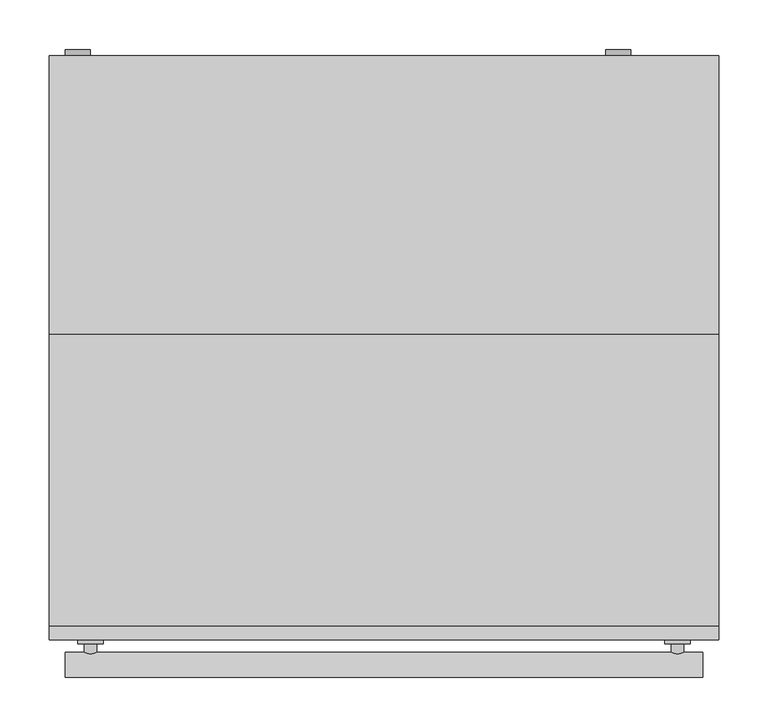
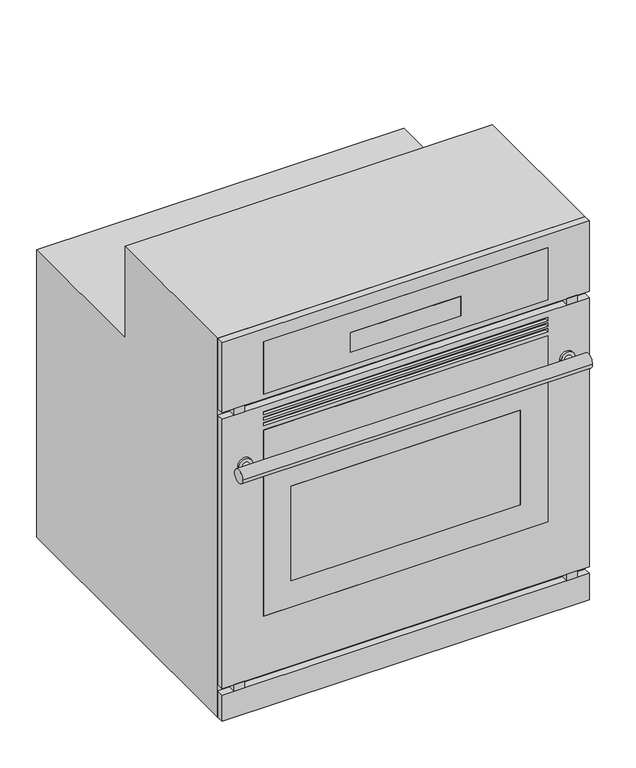
"""IFC4 building model written with IfcOpenShell, lengths in millimetres: proxy geometry, Ovens_Built-In-Wall-Single_GE-Monogram_ZEK938SMSS : Ovens_Built-In-Wall-Single_GE-Monogram_ZEK938SMSS."""

from ifc_helpers import new_model, si_unit, point, frame, frame_2d, origin, place, context, project, spatial, polyline, circle_curve, trimmed, segment, composite_curve, outline, extrude, faceted_brep, source, transform, mapped, element, save
from ifc_brep_helpers import plane_surface, cylinder_surface, advanced_brep


def specialty_equipment_95a57712(model_context):
    return source(origin(), model_context, "Body", "SolidModel", [
        advanced_brep(
        [(-309.3357143, -313.0409311, 485.7987745), (-283.9357143, -313.0409311, 485.7987745), (-290.2857143, -313.0409311, 485.7987745), (-302.9857143, -313.0409311, 485.7987745), (-309.3357143, -308.7303349, 485.7987745), (-283.9357143, -308.7303349, 485.7987745), (-302.9857143, -334.1303349, 485.7987745), (-290.2857143, -334.1303349, 485.7987745)],
        [
            (0, 1, circle_curve(frame((-296.6357143, -313.0409311, 485.7987745), z_axis=(0.0, -1.0, 0.0), x_axis=(1.0, 0.0, 0.0)), 12.7)),
            (1, 0, circle_curve(frame((-296.6357143, -313.0409311, 485.7987745), z_axis=(0.0, -1.0, 0.0), x_axis=(1.0, 0.0, 0.0)), 12.7)),
            (2, 3, circle_curve(frame((-296.6357143, -313.0409311, 485.7987745), z_axis=(0.0, 1.0, 0.0), x_axis=(1.0, 0.0, 0.0)), 6.35)),
            (3, 2, circle_curve(frame((-296.6357143, -313.0409311, 485.7987745), z_axis=(0.0, 1.0, 0.0), x_axis=(1.0, 0.0, 0.0)), 6.35)),
            (4, 5, circle_curve(frame((-296.6357143, -308.7303349, 485.7987745), z_axis=(0.0, 1.0, 0.0), x_axis=(1.0, 0.0, 0.0)), 12.7)),
            (5, 4, circle_curve(frame((-296.6357143, -308.7303349, 485.7987745), z_axis=(0.0, 1.0, 0.0), x_axis=(1.0, 0.0, 0.0)), 12.7)),
            (0, 4),
            (5, 1),
            (6, 7, circle_curve(frame((-296.6357143, -334.1303349, 485.7987745), z_axis=(0.0, -1.0, 0.0), x_axis=(1.0, 0.0, 0.0)), 6.35)),
            (7, 6, circle_curve(frame((-296.6357143, -334.1303349, 485.7987745), z_axis=(0.0, -1.0, 0.0), x_axis=(1.0, 0.0, 0.0)), 6.35)),
            (6, 3),
            (2, 7),
        ],
        [
            plane_surface(frame((-283.9357143, -313.0409311, 485.7987745), z_axis=(0.0, -1.0, 0.0), x_axis=(0.0, 0.0, 1.0))),
            plane_surface(frame((-283.9357143, -308.7303349, 485.7987745), z_axis=(0.0, 1.0, 0.0), x_axis=(0.0, 0.0, -1.0))),
            cylinder_surface(frame((-296.6357143, -308.7303349, 485.7987745), z_axis=(0.0, -1.0, 0.0), x_axis=(1.0, 0.0, 0.0)), 12.7),
            plane_surface(frame((-290.2857143, -334.1303349, 485.7987745), z_axis=(0.0, -1.0, 0.0), x_axis=(0.0, 0.0, 1.0))),
            cylinder_surface(frame((-296.6357143, -308.7303349, 485.7987745), z_axis=(0.0, -1.0, 0.0), x_axis=(1.0, 0.0, 0.0)), 6.35),
        ],
        [
            (0, [[1, 2], [3, 4]]),
            (1, [[5, 6]]),
            (2, [[-1, 7, -6, 8]]),
            (2, [[-2, -8, -5, -7]]),
            (3, [[9, 10]]),
            (4, [[-9, 11, -3, 12]]),
            (4, [[-10, -12, -4, -11]]),
        ],
    ),
        advanced_brep(
        [(283.9357143, -313.0409311, 485.7987745), (309.3357143, -313.0409311, 485.7987745), (302.9857143, -313.0409311, 485.7987745), (290.2857143, -313.0409311, 485.7987745), (283.9357143, -308.7303349, 485.7987745), (309.3357143, -308.7303349, 485.7987745), (290.2857143, -334.1303349, 485.7987745), (302.9857143, -334.1303349, 485.7987745)],
        [
            (0, 1, circle_curve(frame((296.6357143, -313.0409311, 485.7987745), z_axis=(0.0, -1.0, 0.0), x_axis=(1.0, 0.0, 0.0)), 12.7)),
            (1, 0, circle_curve(frame((296.6357143, -313.0409311, 485.7987745), z_axis=(0.0, -1.0, 0.0), x_axis=(1.0, 0.0, 0.0)), 12.7)),
            (2, 3, circle_curve(frame((296.6357143, -313.0409311, 485.7987745), z_axis=(0.0, 1.0, 0.0), x_axis=(1.0, 0.0, 0.0)), 6.35)),
            (3, 2, circle_curve(frame((296.6357143, -313.0409311, 485.7987745), z_axis=(0.0, 1.0, 0.0), x_axis=(1.0, 0.0, 0.0)), 6.35)),
            (4, 5, circle_curve(frame((296.6357143, -308.7303349, 485.7987745), z_axis=(0.0, 1.0, 0.0), x_axis=(1.0, 0.0, 0.0)), 12.7)),
            (5, 4, circle_curve(frame((296.6357143, -308.7303349, 485.7987745), z_axis=(0.0, 1.0, 0.0), x_axis=(1.0, 0.0, 0.0)), 12.7)),
            (0, 4),
            (5, 1),
            (6, 7, circle_curve(frame((296.6357143, -334.1303349, 485.7987745), z_axis=(0.0, -1.0, 0.0), x_axis=(1.0, 0.0, 0.0)), 6.35)),
            (7, 6, circle_curve(frame((296.6357143, -334.1303349, 485.7987745), z_axis=(0.0, -1.0, 0.0), x_axis=(1.0, 0.0, 0.0)), 6.35)),
            (6, 3),
            (2, 7),
        ],
        [
            plane_surface(frame((-283.9357143, -313.0409311, 485.7987745), z_axis=(0.0, -1.0, 0.0), x_axis=(0.0, 0.0, 1.0))),
            plane_surface(frame((-283.9357143, -308.7303349, 485.7987745), z_axis=(0.0, 1.0, 0.0), x_axis=(0.0, 0.0, -1.0))),
            cylinder_surface(frame((296.6357143, -308.7303349, 485.7987745), z_axis=(0.0, -1.0, 0.0), x_axis=(1.0, 0.0, 0.0)), 12.7),
            plane_surface(frame((-290.2857143, -334.1303349, 485.7987745), z_axis=(0.0, -1.0, 0.0), x_axis=(0.0, 0.0, 1.0))),
            cylinder_surface(frame((296.6357143, -308.7303349, 485.7987745), z_axis=(0.0, -1.0, 0.0), x_axis=(1.0, 0.0, 0.0)), 6.35),
        ],
        [
            (0, [[1, 2], [3, 4]]),
            (1, [[5, 6]]),
            (2, [[-1, 7, -6, 8]]),
            (2, [[-2, -8, -5, -7]]),
            (3, [[9, 10]]),
            (4, [[-9, 11, -3, 12]]),
            (4, [[-10, -12, -4, -11]]),
        ],
    ),
        extrude(outline(composite_curve([segment(trimmed(circle_curve(frame_2d((-334.1303349, 486.3026594)), 12.7), [point((-346.8303349, 486.3026594))], [point((-321.4303349, 486.3026594))], False, "CARTESIAN"), True, "CONTINUOUS"), segment(trimmed(circle_curve(frame_2d((-334.1303349, 486.3026594)), 12.7), [point((-321.4303349, 486.3026594))], [point((-346.8303349, 486.3026594))], False, "CARTESIAN"), True, "CONTINUOUS")], self_intersect=False)), frame((-322.0357143, 0.0, 0.0), z_axis=(1.0, 0.0, 0.0), x_axis=(0.0, 1.0, 0.0)), (0.0, 0.0, 1.0), 644.0714286),
        extrude(outline(polyline([(101.6, -308.7303349), (-101.6, -308.7303349), (-101.6, -295.275), (101.6, -295.275), (101.6, -308.7303349)])), frame((0.0, 0.0, 635.0), z_axis=(0.0, 0.0, 1.0), x_axis=(1.0, 0.0, 0.0)), (0.0, 0.0, 1.0), 38.1),
        extrude(outline(polyline([(211.1375, -308.7303349), (-211.1375, -308.7303349), (-211.1375, -295.275), (211.1375, -295.275), (211.1375, -308.7303349)])), frame((0.0, 0.0, 228.6), z_axis=(0.0, 0.0, 1.0), x_axis=(1.0, 0.0, 0.0)), (0.0, 0.0, 1.0), 184.15),
        extrude(outline(polyline([(711.2, 261.9375), (711.2, -261.9375), (609.6, -261.9375), (609.6, 261.9375), (711.2, 261.9375)]), holes=[polyline([(673.1, 101.6), (635.0, 101.6), (635.0, -101.6), (673.1, -101.6), (673.1, 101.6)])]), frame((0.0, -308.7303349, 0.0), z_axis=(0.0, 1.0, 0.0), x_axis=(0.0, 0.0, 1.0)), (0.0, 0.0, 1.0), 13.4553349),
        extrude(outline(polyline([(539.75, -261.9375), (177.8, -261.9375), (177.8, 261.9375), (539.75, 261.9375), (539.75, -261.9375)]), holes=[polyline([(228.6, 211.1375), (228.6, -211.1375), (412.75, -211.1375), (412.75, 211.1375), (228.6, 211.1375)])]), frame((0.0, -308.7303349, 0.0), z_axis=(0.0, 1.0, 0.0), x_axis=(0.0, 0.0, 1.0)), (0.0, 0.0, 1.0), 13.4553349),
        extrude(outline(polyline([(-296.970361, -308.7303349), (-316.020361, -308.7303349), (-316.020361, -295.275), (-296.970361, -295.275), (-296.970361, -308.7303349)])), frame((0.0, 0.0, 50.8), z_axis=(0.0, 0.0, 1.0), x_axis=(1.0, 0.0, 0.0)), (0.0, 0.0, 1.0), 12.7),
        extrude(outline(polyline([(316.020361, -308.7303349), (296.970361, -308.7303349), (296.970361, -295.275), (316.020361, -295.275), (316.020361, -308.7303349)])), frame((0.0, 0.0, 50.8), z_axis=(0.0, 0.0, 1.0), x_axis=(1.0, 0.0, 0.0)), (0.0, 0.0, 1.0), 12.7),
        extrude(outline(polyline([(-296.970361, -308.7303349), (-316.020361, -308.7303349), (-316.020361, -295.275), (-296.970361, -295.275), (-296.970361, -308.7303349)])), frame((0.0, 0.0, 587.3987745), z_axis=(0.0, 0.0, 1.0), x_axis=(1.0, 0.0, 0.0)), (0.0, 0.0, 1.0), 12.7),
        extrude(outline(polyline([(316.020361, -308.7303349), (296.970361, -308.7303349), (296.970361, -295.275), (316.020361, -295.275), (316.020361, -308.7303349)])), frame((0.0, 0.0, 587.3987745), z_axis=(0.0, 0.0, 1.0), x_axis=(1.0, 0.0, 0.0)), (0.0, 0.0, 1.0), 12.7),
        faceted_brep([(-338.1375, -308.7303349, 736.6), (-338.1375, -308.7303349, 600.0987745), (338.1375, -308.7303349, 600.0987745), (338.1375, -308.7303349, 736.6), (-261.9375, -308.7303349, 711.2), (261.9375, -308.7303349, 711.2), (261.9375, -308.7303349, 609.6), (-261.9375, -308.7303349, 609.6), (-338.1375, -295.275, 736.6), (338.1375, -295.275, 736.6), (338.1375, -295.275, 600.0987745), (-338.1375, -295.275, 600.0987745), (-261.9375, -295.275, 711.2), (-261.9375, -295.275, 609.6), (261.9375, -295.275, 609.6), (261.9375, -295.275, 711.2)], [[[0, 1, 2, 3], [4, 5, 6, 7]], [[8, 9, 10, 11], [12, 13, 14, 15]], [[1, 0, 8, 11]], [[2, 1, 11, 10]], [[3, 2, 10, 9]], [[0, 3, 9, 8]], [[5, 4, 12, 15]], [[6, 5, 15, 14]], [[7, 6, 14, 13]], [[4, 7, 13, 12]]]),
        faceted_brep([(338.1375, -308.7303349, 0.0), (338.1375, -308.7303349, 50.8), (-338.1375, -308.7303349, 50.8), (-338.1375, -308.7303349, 0.0), (338.1375, -295.275, 0.0), (-338.1375, -295.275, 0.0), (-338.1375, -295.275, 50.8), (338.1375, -295.275, 50.8)], [[[0, 1, 2, 3]], [[4, 5, 6, 7]], [[1, 0, 4, 7]], [[2, 1, 7, 6]], [[3, 2, 6, 5]], [[0, 3, 5, 4]]]),
        faceted_brep([(-338.1375, -308.7303349, 63.5), (338.1375, -308.7303349, 63.5), (338.1375, -308.7303349, 587.3987745), (-338.1375, -308.7303349, 587.3987745), (-261.9375, -308.7303349, 558.6731386), (-261.9375, -308.7303349, 565.0231386), (261.9375, -308.7303349, 565.0231386), (261.9375, -308.7303349, 558.6731386), (-261.9375, -308.7303349, 177.8), (-261.9375, -308.7303349, 539.75), (261.9375, -308.7303349, 539.75), (261.9375, -308.7303349, 177.8), (-261.9375, -308.7303349, 548.0044527), (-261.9375, -308.7303349, 554.3544527), (261.9375, -308.7303349, 554.3544527), (261.9375, -308.7303349, 548.0044527), (-261.9375, -308.7303349, 569.3418245), (-261.9375, -308.7303349, 575.6918245), (261.9375, -308.7303349, 575.6918245), (261.9375, -308.7303349, 569.3418245), (-338.1375, -295.275, 63.5), (-338.1375, -295.275, 587.3987745), (338.1375, -295.275, 587.3987745), (338.1375, -295.275, 63.5), (261.9375, -295.275, 177.8), (261.9375, -295.275, 539.75), (-261.9375, -295.275, 539.75), (-261.9375, -295.275, 177.8), (261.9375, -302.3803349, 565.0231386), (261.9375, -302.3803349, 558.6731386), (261.9375, -302.3803349, 554.3544527), (261.9375, -302.3803349, 548.0044527), (261.9375, -302.3803349, 575.6918245), (261.9375, -302.3803349, 569.3418245), (-261.9375, -302.3803349, 558.6731386), (-261.9375, -302.3803349, 565.0231386), (-261.9375, -302.3803349, 548.0044527), (-261.9375, -302.3803349, 554.3544527), (-261.9375, -302.3803349, 569.3418245), (-261.9375, -302.3803349, 575.6918245)], [[[0, 1, 2, 3], [4, 5, 6, 7], [8, 9, 10, 11], [12, 13, 14, 15], [16, 17, 18, 19]], [[20, 21, 22, 23], [24, 25, 26, 27]], [[1, 0, 20, 23]], [[2, 1, 23, 22]], [[3, 2, 22, 21]], [[7, 6, 28, 29]], [[15, 14, 30, 31]], [[19, 18, 32, 33]], [[24, 11, 10, 25]], [[8, 11, 24, 27]], [[5, 4, 34, 35]], [[13, 12, 36, 37]], [[17, 16, 38, 39]], [[8, 27, 26, 9]], [[0, 3, 21, 20]], [[18, 17, 39, 32]], [[32, 39, 38, 33]], [[33, 38, 16, 19]], [[6, 5, 35, 28]], [[28, 35, 34, 29]], [[29, 34, 4, 7]], [[14, 13, 37, 30]], [[30, 37, 36, 31]], [[31, 36, 12, 15]], [[26, 25, 10, 9]]]),
        extrude(outline(polyline([(-295.275, 0.0), (-295.275, 736.6), (0.0, 736.6), (0.0, 558.8), (281.8196651, 558.8), (281.8196651, 0.0), (-295.275, 0.0)])), frame((-338.1375, 0.0, 0.0), z_axis=(1.0, 0.0, 0.0), x_axis=(0.0, 1.0, 0.0)), (0.0, 0.0, 1.0), 676.275),
        extrude(outline(composite_curve([segment(trimmed(circle_curve(frame_2d((314.6288473, -309.3887314)), 12.7), [point((314.6288473, -296.6887314))], [point((314.6288473, -322.0887314))], False, "CARTESIAN"), True, "CONTINUOUS"), segment(trimmed(circle_curve(frame_2d((314.6288473, -309.3887314)), 12.7), [point((314.6288473, -322.0887314))], [point((314.6288473, -296.6887314))], False, "CARTESIAN"), True, "CONTINUOUS")], self_intersect=False)), frame((0.0, 281.8196651, 0.0), z_axis=(0.0, 1.0, 0.0), x_axis=(0.0, 0.0, 1.0)), (0.0, 0.0, 1.0), 6.35),
        extrude(outline(composite_curve([segment(trimmed(circle_curve(frame_2d((314.6288473, 236.7112686)), 12.7), [point((314.6288473, 249.4112686))], [point((314.6288473, 224.0112686))], False, "CARTESIAN"), True, "CONTINUOUS"), segment(trimmed(circle_curve(frame_2d((314.6288473, 236.7112686)), 12.7), [point((314.6288473, 224.0112686))], [point((314.6288473, 249.4112686))], False, "CARTESIAN"), True, "CONTINUOUS")], self_intersect=False)), frame((0.0, 281.8196651, 0.0), z_axis=(0.0, 1.0, 0.0), x_axis=(0.0, 0.0, 1.0)), (0.0, 0.0, 1.0), 6.35),
    ])


if __name__ == "__main__":
    model = new_model("IFC4")
    model_context = context("Model", 3, world=origin())
    ifc_project = project(units=[si_unit("LENGTHUNIT", "METRE", prefix="MILLI")], contexts=[model_context])
    site = spatial("IfcSite", under=ifc_project)
    building = spatial("IfcBuilding", under=site)
    placement = place(None, origin())
    specialty_equipment_shape = specialty_equipment_95a57712(model_context)
    element("IfcBuildingElementProxy", 1, Name="Ovens_Built-In-Wall-Single_GE-Monogram_ZEK938SMSS : Ovens_Built-In-Wall-Single_GE-Monogram_ZEK938SMSS", ObjectType="Ovens_Built-In-Wall-Single_GE-Monogram_ZEK938SMSS : Ovens_Built-In-Wall-Single_GE-Monogram_ZEK938SMSS", at=placement, inside=building, context=model_context, shape_type="MappedRepresentation", body=[
        mapped(specialty_equipment_shape, transform((0.0, 0.0, 0.0), x_axis=(1.0, 0.0, 0.0), y_axis=(0.0, 1.0, 0.0), z_axis=(0.0, 0.0, 1.0))),
    ])
    save(model, "model.ifc")

# Revit data of these elements
# Type "Ovens_Built-In-Wall-Single_GE-Monogram_ZEK938SMSS : Ovens_Built-In-Wall-Single_GE-Monogram_ZEK938SMSS"
#   COBie.Type.CreatedBy = "design@eagle.com"
#   COBie.Type.CreatedOn = "2016-10-27T05:31:12"
#   COBie.Type.Name = "Ovens_Built-In-Wall-Single_GE-Monogram_ZEK938SMSS_Ovens_Built-In-Wall-Single_GE-Monogram_ZEK938SMSS"
#   COBie.Type.Category = "23-40 40 14 17 11 : Cookers, Ovens, Stoves"
#   COBie.Type.Description = "Ovens_Built-In-Wall-Single_GE-Monogram_ZEK938SMSS_Ovens_Built-In-Wall-Single_GE-Monogram_ZEK938SMSS"
#   COBie.Type.Manufacturer = "info@geappliances.com"
#   COBie.Type.ModelNumber = "As Specified in 11 30 00"
#   URL = "http://www.geappliances.com/"
#   Test Data = "http://www.geappliances.com/service_and_support/search.htm"
#   Specification = "http://www.arcat.com/sdspecs/htm/11450gea.htm"
#   SpecWizard = "http://www.arcat.com/specwizard/11450gea/index.htm?mf=&coid=32703"
#   Send Message = "http://www.arcat.com/users.pl?action=UserEmail&company=GE%20Appliances&coid=32703&rep=114&fax=502-452-0620&mf="
#   Sales Information = "http://www.geappliances.com/buy/"
#   Revision = "R1_02-2011"
#   Product Properties = "http://www.arcat.com/bim/bim_info.pl?fn=GEAppliances"
#   Product Data = "http://www.arcat.com/arcatcos/cos32/arc32703.html"
#   Model = "As Specified in 11 30 00"
#   Manufacturer Website = "http://www.geappliances.com/"
#   Manufacturer Phone - Toll Free = "800-626-2000"
#   Manufacturer Phone = "502-452-3346"
#   Manufacturer Fax = "502-452-0620"
#   Manufacturer Address = "Appliance Park AP4-109, Louisville, KY 40225"
#   Manufacturer = "info@geappliances.com"
#   Keynote = "11 30 00"
#   Installation-Fabrication = "http://www.geappliances.com/service_and_support/literature/"
#   Installation Phase = ""
#   Heat Source = ""
#   Green Building-LEED = "http://www.geappliances.com/energy-star-appliances/"
#   ENERGYSTAR Qualified = ""
#   Drawn By = "Sumex Design, Inc. / Robert S. Weygant, CSI, CDT, SCIP"
#   Description = "Residential Appliance as Specified in 11 30 00"
#   Copyright = "©Arcat Inc."
#   Cooktop Type = ""
#   Cooking Technology = ""
#   Construction Details = "http://www.geappliances.com/design_center/"
#   Building Codes = "http://www.geappliances.com/service_and_support/search.htm"
#   Assembly Code = "E1090400"
#   COBie.Type.ReplacementCost = 0
#   offset [instance default] = 0' - 0"
#   Handle Width [instance default] = 2' - 1.35714"
#   Voltage_MEP = 120 V
#   Unit Width = 2' - 2 5/8"
#   Unit Height = 2' - 5"
#   Unit Depth = 1' - 11 1/4"
#   MEP Apparent Power = 60 VA
#   MEP Amperage = 0.5 A
#   HWRad = 0' - 0 1/4"
#   GasRad = 0' - 0 1/4"
#   DrainRad = 0' - 0 5/8"
#   Connection Dia HW = 0' - 0 1/2"
#   Connection Dia Gas = 0' - 0 1/2"
#   Connection Dia DWV = 0' - 1 1/4"
#   Connection Dia CW = 0' - 0 1/2"
#   CWRad = 0' - 0 1/4"
#   COBie.Type = yes
#   Warranty Duration (Years) = 5
#   Self Cleaning = yes
#   Maintenance Schedule (Months) = 0
#   Expected Lifespan (Years) = 25
#   ADA Compliant = yes
#   Handle Finish = none
#   Glass = Glass
#   Exterior Finish = ARCAT - Finish - Stainless steel
# Element 1 (IfcBuildingElementProxy, "Ovens_Built-In-Wall-Single_GE-Monogram_ZEK938SMSS : Ovens_Built-In-Wall-Single_GE-Monogram_ZEK938SMSS")
#   Materials on its faces: "ARCAT - Finish - Stainless steel", "Glass", "Gas", "Connector"
# Materials
#   "Glass": class "Glass", colour RGB 0 128 192, transparency 0.75, Description = "Soda Lime Glass", Cost = 0
#   "ARCAT - Finish - Stainless steel": class "Unassigned", colour RGB 244 244 244, transparency 0, Keynote = "09910", Model = "Generic", Manufacturer = "Generic", Description = "Paints"
#   "Gas": class "Miscellaneous", colour RGB 255 0 255, transparency 0
#   "Connector": class "Miscellaneous", colour RGB 255 255 0, transparency 0
